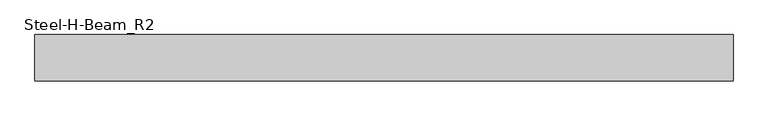
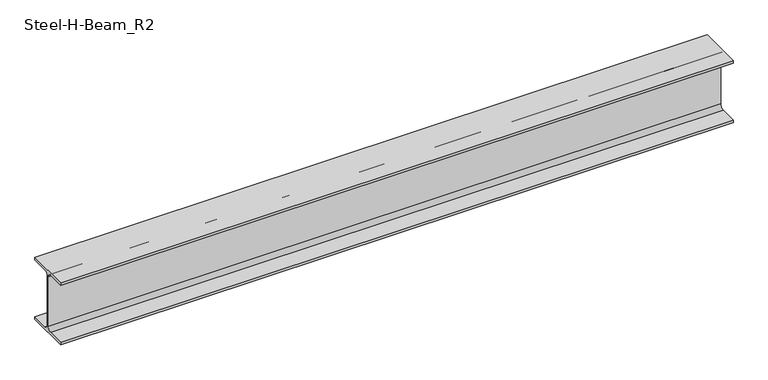
"""IFC4 building model written with IfcOpenShell, lengths in millimetres: beam geometry, Steel-H-Beam_R2 : BM121_H-294×200x8x12_SB1."""

import ifcopenshell
import ifcopenshell.guid

model = None  # the IFC model being written
_history = None  # IfcOwnerHistory: only IFC2X3 demands one
_inside = {}  # id of a spatial element -> (the spatial element, [elements in it])
_under = {}  # id of a project, library or spatial element -> (it, [spatial elements below it])
_declared = {}  # id of a project -> (the project, [libraries it declares])
_typed = {}  # id of a type object -> (the type object, [elements of that type])
_made_of = {}  # id of a material, layer set ... -> (it, [elements and type objects made of it])


def new_model(schema):
    """Start an empty IFC model of exactly this schema.

    Asked for "IFC4X3", IfcOpenShell would pick the latest addendum, in which some entities
    have other attributes; the version numbers below select the first issue.
    IFC2X3 requires an IfcOwnerHistory on every rooted entity: one is made here for all.
    """
    global model, _history
    if schema == "IFC4X3":
        model = ifcopenshell.file(schema_version=(4, 3, 0, 0))
    else:
        model = ifcopenshell.file(schema=schema)
    _inside.clear()
    _under.clear()
    _declared.clear()
    _typed.clear()
    _made_of.clear()
    _history = None
    if model.schema == "IFC2X3":
        org = make("IfcOrganization", Name="unknown")
        user = make(
            "IfcPersonAndOrganization",
            ThePerson=make("IfcPerson", FamilyName="unknown"),
            TheOrganization=org,
        )
        app = make(
            "IfcApplication",
            ApplicationDeveloper=org,
            Version="unknown",
            ApplicationFullName="unknown",
            ApplicationIdentifier="unknown",
        )
        _history = make(
            "IfcOwnerHistory",
            OwningUser=user,
            OwningApplication=app,
            ChangeAction="ADDED",
            CreationDate=0,
        )
    return model


def make(cls, **values):
    """One entity of the class cls with the attributes given. An attribute that is None is left unset."""
    return model.create_entity(
        cls, **{name: value for name, value in values.items() if value is not None}
    )


def rooted(cls, **values):
    """An entity with a GlobalId (a new one), such as an element, a storey or a relation."""
    return make(cls, GlobalId=ifcopenshell.guid.new(), OwnerHistory=_history, **values)


def si_unit(unit_type, name, prefix=None):
    """IfcSIUnit, for example si_unit("LENGTHUNIT", "METRE", prefix="MILLI")."""
    return make("IfcSIUnit", UnitType=unit_type, Prefix=prefix, Name=name)


def assignment(units):
    """IfcUnitAssignment: the units of a project."""
    return None if units is None else make("IfcUnitAssignment", Units=units)


def point(xyz):
    """IfcCartesianPoint."""
    return None if xyz is None else make("IfcCartesianPoint", Coordinates=xyz)


def direction(xyz):
    """IfcDirection."""
    return None if xyz is None else make("IfcDirection", DirectionRatios=xyz)


def frame(location, z_axis=None, x_axis=None):
    """IfcAxis2Placement3D, a coordinate frame: its origin and axes. An axis left out is left unset."""
    return make(
        "IfcAxis2Placement3D",
        Location=point(location),
        Axis=direction(z_axis),
        RefDirection=direction(x_axis),
    )


def frame_2d(location, x_axis=None):
    """IfcAxis2Placement2D, a coordinate frame in the plane: its origin and x axis."""
    return make(
        "IfcAxis2Placement2D", Location=point(location), RefDirection=direction(x_axis)
    )


def origin():
    """The frame at (0, 0, 0) with its axes left unset."""
    return frame((0.0, 0.0, 0.0))


def place(relative_to, where):
    """IfcLocalPlacement: puts the frame where relative to a parent placement (None: the world)."""
    return make(
        "IfcLocalPlacement", PlacementRelTo=relative_to, RelativePlacement=where
    )


def context(
    kind, dimensions, precision=None, world=None, true_north=None, identifier=None
):
    """IfcGeometricRepresentationContext, for example the 3D "Model" context."""
    return make(
        "IfcGeometricRepresentationContext",
        ContextIdentifier=identifier,
        ContextType=kind,
        CoordinateSpaceDimension=dimensions,
        Precision=precision,
        WorldCoordinateSystem=world,
        TrueNorth=true_north,
    )


def project(units=None, contexts=None):
    """IfcProject with its units and contexts."""
    return rooted(
        "IfcProject",
        Name="project",
        RepresentationContexts=contexts,
        UnitsInContext=assignment(units),
    )


def spatial(cls, under=None, at=None, **own):
    """A site, building, storey or space (cls), placed at a placement, below another one or the project."""
    s = rooted(cls, ObjectPlacement=at, **own)
    if under is not None:
        _under.setdefault(under.id(), (under, []))[1].append(s)
    return s


def polyline(points):
    """IfcPolyline through the points."""
    return make("IfcPolyline", Points=[point(p) for p in points])


def circle_curve(where, radius):
    """IfcCircle in the frame where."""
    return make("IfcCircle", Position=where, Radius=radius)


def trimmed(basis, trim1, trim2, sense, master):
    """IfcTrimmedCurve: the piece of a basis curve between two trims."""
    return make(
        "IfcTrimmedCurve",
        BasisCurve=basis,
        Trim1=trim1,
        Trim2=trim2,
        SenseAgreement=sense,
        MasterRepresentation=master,
    )


def segment(curve, same_sense, transition):
    """IfcCompositeCurveSegment."""
    return make(
        "IfcCompositeCurveSegment",
        Transition=transition,
        SameSense=same_sense,
        ParentCurve=curve,
    )


def composite_curve(segments, self_intersect=None):
    """IfcCompositeCurve: segments joined end to end."""
    return make("IfcCompositeCurve", Segments=segments, SelfIntersect=self_intersect)


def outline(outer, holes=None, kind="AREA"):
    """IfcArbitraryClosedProfileDef: a profile drawn as a closed curve; with holes, ...WithVoids."""
    if holes is None:
        return make("IfcArbitraryClosedProfileDef", ProfileType=kind, OuterCurve=outer)
    return make(
        "IfcArbitraryProfileDefWithVoids",
        ProfileType=kind,
        OuterCurve=outer,
        InnerCurves=holes,
    )


def extrude(swept, where, along, depth):
    """IfcExtrudedAreaSolid: the profile swept, set in the frame where, extruded along a direction by depth."""
    return make(
        "IfcExtrudedAreaSolid",
        SweptArea=swept,
        Position=where,
        ExtrudedDirection=direction(along),
        Depth=depth,
    )


def shape(context_of_items, identifier, shape_type, items):
    """IfcShapeRepresentation: the items that make up one representation, for example the "Body"."""
    return make(
        "IfcShapeRepresentation",
        ContextOfItems=context_of_items,
        RepresentationIdentifier=identifier,
        RepresentationType=shape_type,
        Items=items,
    )


def source(mapping_origin, context_of_items, identifier, shape_type, items):
    """IfcRepresentationMap: a shape defined once, which mapped items show again and again."""
    return make(
        "IfcRepresentationMap",
        MappingOrigin=mapping_origin,
        MappedRepresentation=shape(context_of_items, identifier, shape_type, items),
    )


def transform(
    local_origin,
    x_axis=None,
    y_axis=None,
    z_axis=None,
    scale=None,
    scale2=None,
    scale3=None,
    uniform=True,
):
    """IfcCartesianTransformationOperator3D, or its non-uniform kind. x_axis, y_axis, z_axis: its Axis1, 2, 3."""
    if uniform:
        return make(
            "IfcCartesianTransformationOperator3D",
            Axis1=direction(x_axis),
            Axis2=direction(y_axis),
            LocalOrigin=point(local_origin),
            Scale=scale,
            Axis3=direction(z_axis),
        )
    return make(
        "IfcCartesianTransformationOperator3DnonUniform",
        Axis1=direction(x_axis),
        Axis2=direction(y_axis),
        LocalOrigin=point(local_origin),
        Scale=scale,
        Axis3=direction(z_axis),
        Scale2=scale2,
        Scale3=scale3,
    )


def mapped(mapping_source, mapping_target):
    """IfcMappedItem: shows the shape of a source again, moved by a transform."""
    return make(
        "IfcMappedItem", MappingSource=mapping_source, MappingTarget=mapping_target
    )


def made_of(thing, what):
    """Note that an element or type object is made of a material, layer set ...; save() writes the relation."""
    if what is not None:
        _made_of.setdefault(what.id(), (what, []))[1].append(thing)
    return thing


def element(
    cls,
    number,
    at=None,
    inside=None,
    cuts=None,
    type_object=None,
    material=None,
    context=None,
    identifier="Body",
    shape_type=None,
    held_by="IfcProductDefinitionShape",
    body=None,
    shapes=None,
    **own,
):
    """One element of the class cls, such as IfcWall. Its Tag is "e" and its number.

    at: its placement. inside: the storey or other place that contains it. cuts: it is an
    opening in that element (IfcRelVoidsElement). A single representation is given by context,
    identifier, shape_type and body (its items); several are given by shapes. held_by: the class
    of the entity that holds the representations. save() writes the other relations.
    """
    e = rooted(cls, Tag="e%d" % number, ObjectPlacement=at, **own)
    if body is not None:
        shapes = [shape(context, identifier, shape_type, body)]
    if shapes is not None:
        e.Representation = make(held_by, Representations=shapes)
    if inside is not None:
        _inside.setdefault(inside.id(), (inside, []))[1].append(e)
    if cuts is not None:
        rooted(
            "IfcRelVoidsElement", RelatingBuildingElement=cuts, RelatedOpeningElement=e
        )
    if type_object is not None:
        _typed.setdefault(type_object.id(), (type_object, []))[1].append(e)
    return made_of(e, material)


def aggregate(whole, parts):
    """IfcRelAggregates: a whole, such as a stair, and the parts it consists of."""
    return rooted("IfcRelAggregates", RelatingObject=whole, RelatedObjects=parts)


def save(model, path):
    """Write the relations noted so far, then the file.

    IfcRelAggregates (storeys below a building ...), IfcRelContainedInSpatialStructure (elements
    in a storey), IfcRelDefinesByType, IfcRelAssociatesMaterial and IfcRelDeclares: one each for
    every whole, place, type object, material and project.
    """
    for whole, parts in _under.values():
        aggregate(whole, parts)
    for where, things in _inside.values():
        rooted(
            "IfcRelContainedInSpatialStructure",
            RelatedElements=things,
            RelatingStructure=where,
        )
    for kind, things in _typed.values():
        rooted("IfcRelDefinesByType", RelatedObjects=things, RelatingType=kind)
    for what, things in _made_of.values():
        rooted("IfcRelAssociatesMaterial", RelatedObjects=things, RelatingMaterial=what)
    for by, libraries in _declared.values():
        rooted("IfcRelDeclares", RelatingContext=by, RelatedDefinitions=libraries)
    model.write(path)


def steel_h_beam_r2_827bf599(model_context):
    return source(origin(), model_context, "Body", "SweptSolid", [
        extrude(outline(composite_curve([segment(polyline([(100.0, -135.0), (100.0, -147.0), (-100.0, -147.0), (-100.0, -135.0), (-22.0, -135.0)]), True, "CONTINUOUS"), segment(trimmed(circle_curve(frame_2d((-22.0, -117.0)), 18.0), [point((-22.0, -135.0))], [point((-4.0, -117.0))], True, "CARTESIAN"), True, "CONTINUOUS"), segment(polyline([(-4.0, -117.0), (-4.0, 117.0)]), True, "CONTINUOUS"), segment(trimmed(circle_curve(frame_2d((-22.0, 117.0)), 18.0), [point((-4.0, 117.0))], [point((-22.0, 135.0))], True, "CARTESIAN"), True, "CONTINUOUS"), segment(polyline([(-22.0, 135.0), (-100.0, 135.0), (-100.0, 147.0), (100.0, 147.0), (100.0, 135.0), (22.0, 135.0)]), True, "CONTINUOUS"), segment(trimmed(circle_curve(frame_2d((22.0, 117.0)), 18.0), [point((22.0, 135.0))], [point((4.0, 117.0))], True, "CARTESIAN"), True, "CONTINUOUS"), segment(polyline([(4.0, 117.0), (4.0, -117.0)]), True, "CONTINUOUS"), segment(trimmed(circle_curve(frame_2d((22.0, -117.0)), 18.0), [point((4.0, -117.0))], [point((22.0, -135.0))], True, "CARTESIAN"), True, "CONTINUOUS"), segment(polyline([(22.0, -135.0), (100.0, -135.0)]), True, "CONTINUOUS")], self_intersect=False)), frame((-1512.3, 0.0, 0.0), z_axis=(1.0, 0.0, 0.0), x_axis=(0.0, 1.0, 0.0)), (0.0, 0.0, 1.0), 3012.3),
    ])


if __name__ == "__main__":
    model = new_model("IFC4")
    model_context = context("Model", 3, world=origin())
    ifc_project = project(units=[si_unit("LENGTHUNIT", "METRE", prefix="MILLI")], contexts=[model_context])
    site = spatial("IfcSite", under=ifc_project)
    building = spatial("IfcBuilding", under=site)
    placement = place(None, origin())
    steel_h_beam_r2_shape = steel_h_beam_r2_827bf599(model_context)
    element("IfcBeam", 1, ObjectType="Steel-H-Beam_R2 : BM121_H-294×200x8x12_SB1", at=placement, inside=building, context=model_context, shape_type="MappedRepresentation", body=[
        mapped(steel_h_beam_r2_shape, transform((0.0, 0.0, 0.0), x_axis=(1.0, 0.0, 0.0), y_axis=(0.0, 1.0, 0.0), z_axis=(0.0, 0.0, 1.0))),
    ])
    save(model, "model.ifc")

# Revit data of these elements
# Type "Steel-H-Beam_R2 : BM121_H-294×200x8x12_SB1"
#   SteelWeight = "Medium"
#   Surface Area = 1.3411 m²/m
#   Section Area = 72.3812 cm²
#   Mass per Unit Length = 56.8193 kg/m
#   Length [instance default] = 3000 mm
#   B = 200 mm
#   H = 294 mm
#   r = 18 mm
#   tw = 8 mm
#   tf = 12 mm
#   hec_material4 [instance default] = none
#   hec_material3 [instance default] = none
#   hec_material2 [instance default] = none
#   hec_material1 [instance default] = none
#   Structural Material [instance default] = Steel, 45-345
#   Assembly Code = ""
# Element 1 (IfcBeam, "Steel-H-Beam_R2 : BM121_H-294×200x8x12_SB1")
#   Materials on its faces: "Steel, 45-345"
# Materials
#   "Steel, 45-345": class "Metal", colour RGB 189 187 185, transparency 0, Description = "Steel 345 MPa", Cost = 0
